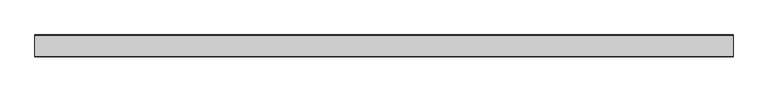
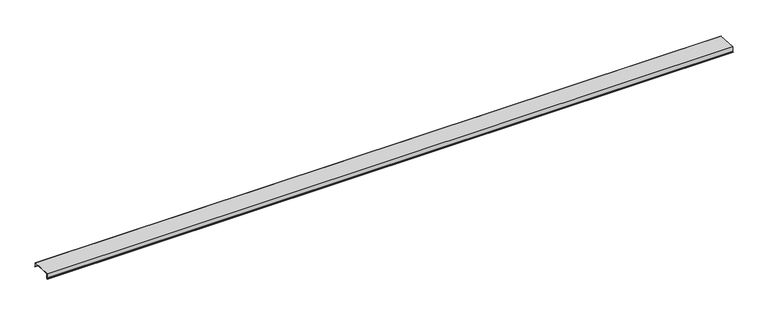
"""IFC4 building model written with IfcOpenShell, lengths in millimetres: proxy geometry, Generic Models 7:Generic Models 1:5:Generic Models 1:5 : Generic Models 7:Generic Models 1:337419:31 : Generic Models 7:Generic Models 1:5:Generic Models 1:5 : Generic Models 7:Generic Models 1:337419:311462."""

import ifcopenshell
import ifcopenshell.guid

model = None  # the IFC model being written
_history = None  # IfcOwnerHistory: only IFC2X3 demands one
_inside = {}  # id of a spatial element -> (the spatial element, [elements in it])
_under = {}  # id of a project, library or spatial element -> (it, [spatial elements below it])
_declared = {}  # id of a project -> (the project, [libraries it declares])
_typed = {}  # id of a type object -> (the type object, [elements of that type])
_made_of = {}  # id of a material, layer set ... -> (it, [elements and type objects made of it])


def new_model(schema):
    """Start an empty IFC model of exactly this schema.

    Asked for "IFC4X3", IfcOpenShell would pick the latest addendum, in which some entities
    have other attributes; the version numbers below select the first issue.
    IFC2X3 requires an IfcOwnerHistory on every rooted entity: one is made here for all.
    """
    global model, _history
    if schema == "IFC4X3":
        model = ifcopenshell.file(schema_version=(4, 3, 0, 0))
    else:
        model = ifcopenshell.file(schema=schema)
    _inside.clear()
    _under.clear()
    _declared.clear()
    _typed.clear()
    _made_of.clear()
    _history = None
    if model.schema == "IFC2X3":
        org = make("IfcOrganization", Name="unknown")
        user = make(
            "IfcPersonAndOrganization",
            ThePerson=make("IfcPerson", FamilyName="unknown"),
            TheOrganization=org,
        )
        app = make(
            "IfcApplication",
            ApplicationDeveloper=org,
            Version="unknown",
            ApplicationFullName="unknown",
            ApplicationIdentifier="unknown",
        )
        _history = make(
            "IfcOwnerHistory",
            OwningUser=user,
            OwningApplication=app,
            ChangeAction="ADDED",
            CreationDate=0,
        )
    return model


def make(cls, **values):
    """One entity of the class cls with the attributes given. An attribute that is None is left unset."""
    return model.create_entity(
        cls, **{name: value for name, value in values.items() if value is not None}
    )


def rooted(cls, **values):
    """An entity with a GlobalId (a new one), such as an element, a storey or a relation."""
    return make(cls, GlobalId=ifcopenshell.guid.new(), OwnerHistory=_history, **values)


def si_unit(unit_type, name, prefix=None):
    """IfcSIUnit, for example si_unit("LENGTHUNIT", "METRE", prefix="MILLI")."""
    return make("IfcSIUnit", UnitType=unit_type, Prefix=prefix, Name=name)


def assignment(units):
    """IfcUnitAssignment: the units of a project."""
    return None if units is None else make("IfcUnitAssignment", Units=units)


def point(xyz):
    """IfcCartesianPoint."""
    return None if xyz is None else make("IfcCartesianPoint", Coordinates=xyz)


def direction(xyz):
    """IfcDirection."""
    return None if xyz is None else make("IfcDirection", DirectionRatios=xyz)


def frame(location, z_axis=None, x_axis=None):
    """IfcAxis2Placement3D, a coordinate frame: its origin and axes. An axis left out is left unset."""
    return make(
        "IfcAxis2Placement3D",
        Location=point(location),
        Axis=direction(z_axis),
        RefDirection=direction(x_axis),
    )


def origin():
    """The frame at (0, 0, 0) with its axes left unset."""
    return frame((0.0, 0.0, 0.0))


def place(relative_to, where):
    """IfcLocalPlacement: puts the frame where relative to a parent placement (None: the world)."""
    return make(
        "IfcLocalPlacement", PlacementRelTo=relative_to, RelativePlacement=where
    )


def context(
    kind, dimensions, precision=None, world=None, true_north=None, identifier=None
):
    """IfcGeometricRepresentationContext, for example the 3D "Model" context."""
    return make(
        "IfcGeometricRepresentationContext",
        ContextIdentifier=identifier,
        ContextType=kind,
        CoordinateSpaceDimension=dimensions,
        Precision=precision,
        WorldCoordinateSystem=world,
        TrueNorth=true_north,
    )


def project(units=None, contexts=None):
    """IfcProject with its units and contexts."""
    return rooted(
        "IfcProject",
        Name="project",
        RepresentationContexts=contexts,
        UnitsInContext=assignment(units),
    )


def spatial(cls, under=None, at=None, **own):
    """A site, building, storey or space (cls), placed at a placement, below another one or the project."""
    s = rooted(cls, ObjectPlacement=at, **own)
    if under is not None:
        _under.setdefault(under.id(), (under, []))[1].append(s)
    return s


def polyline(points):
    """IfcPolyline through the points."""
    return make("IfcPolyline", Points=[point(p) for p in points])


def outline(outer, holes=None, kind="AREA"):
    """IfcArbitraryClosedProfileDef: a profile drawn as a closed curve; with holes, ...WithVoids."""
    if holes is None:
        return make("IfcArbitraryClosedProfileDef", ProfileType=kind, OuterCurve=outer)
    return make(
        "IfcArbitraryProfileDefWithVoids",
        ProfileType=kind,
        OuterCurve=outer,
        InnerCurves=holes,
    )


def extrude(swept, where, along, depth):
    """IfcExtrudedAreaSolid: the profile swept, set in the frame where, extruded along a direction by depth."""
    return make(
        "IfcExtrudedAreaSolid",
        SweptArea=swept,
        Position=where,
        ExtrudedDirection=direction(along),
        Depth=depth,
    )


def shape(context_of_items, identifier, shape_type, items):
    """IfcShapeRepresentation: the items that make up one representation, for example the "Body"."""
    return make(
        "IfcShapeRepresentation",
        ContextOfItems=context_of_items,
        RepresentationIdentifier=identifier,
        RepresentationType=shape_type,
        Items=items,
    )


def source(mapping_origin, context_of_items, identifier, shape_type, items):
    """IfcRepresentationMap: a shape defined once, which mapped items show again and again."""
    return make(
        "IfcRepresentationMap",
        MappingOrigin=mapping_origin,
        MappedRepresentation=shape(context_of_items, identifier, shape_type, items),
    )


def transform(
    local_origin,
    x_axis=None,
    y_axis=None,
    z_axis=None,
    scale=None,
    scale2=None,
    scale3=None,
    uniform=True,
):
    """IfcCartesianTransformationOperator3D, or its non-uniform kind. x_axis, y_axis, z_axis: its Axis1, 2, 3."""
    if uniform:
        return make(
            "IfcCartesianTransformationOperator3D",
            Axis1=direction(x_axis),
            Axis2=direction(y_axis),
            LocalOrigin=point(local_origin),
            Scale=scale,
            Axis3=direction(z_axis),
        )
    return make(
        "IfcCartesianTransformationOperator3DnonUniform",
        Axis1=direction(x_axis),
        Axis2=direction(y_axis),
        LocalOrigin=point(local_origin),
        Scale=scale,
        Axis3=direction(z_axis),
        Scale2=scale2,
        Scale3=scale3,
    )


def mapped(mapping_source, mapping_target):
    """IfcMappedItem: shows the shape of a source again, moved by a transform."""
    return make(
        "IfcMappedItem", MappingSource=mapping_source, MappingTarget=mapping_target
    )


def made_of(thing, what):
    """Note that an element or type object is made of a material, layer set ...; save() writes the relation."""
    if what is not None:
        _made_of.setdefault(what.id(), (what, []))[1].append(thing)
    return thing


def element(
    cls,
    number,
    at=None,
    inside=None,
    cuts=None,
    type_object=None,
    material=None,
    context=None,
    identifier="Body",
    shape_type=None,
    held_by="IfcProductDefinitionShape",
    body=None,
    shapes=None,
    **own,
):
    """One element of the class cls, such as IfcWall. Its Tag is "e" and its number.

    at: its placement. inside: the storey or other place that contains it. cuts: it is an
    opening in that element (IfcRelVoidsElement). A single representation is given by context,
    identifier, shape_type and body (its items); several are given by shapes. held_by: the class
    of the entity that holds the representations. save() writes the other relations.
    """
    e = rooted(cls, Tag="e%d" % number, ObjectPlacement=at, **own)
    if body is not None:
        shapes = [shape(context, identifier, shape_type, body)]
    if shapes is not None:
        e.Representation = make(held_by, Representations=shapes)
    if inside is not None:
        _inside.setdefault(inside.id(), (inside, []))[1].append(e)
    if cuts is not None:
        rooted(
            "IfcRelVoidsElement", RelatingBuildingElement=cuts, RelatedOpeningElement=e
        )
    if type_object is not None:
        _typed.setdefault(type_object.id(), (type_object, []))[1].append(e)
    return made_of(e, material)


def aggregate(whole, parts):
    """IfcRelAggregates: a whole, such as a stair, and the parts it consists of."""
    return rooted("IfcRelAggregates", RelatingObject=whole, RelatedObjects=parts)


def save(model, path):
    """Write the relations noted so far, then the file.

    IfcRelAggregates (storeys below a building ...), IfcRelContainedInSpatialStructure (elements
    in a storey), IfcRelDefinesByType, IfcRelAssociatesMaterial and IfcRelDeclares: one each for
    every whole, place, type object, material and project.
    """
    for whole, parts in _under.values():
        aggregate(whole, parts)
    for where, things in _inside.values():
        rooted(
            "IfcRelContainedInSpatialStructure",
            RelatedElements=things,
            RelatingStructure=where,
        )
    for kind, things in _typed.values():
        rooted("IfcRelDefinesByType", RelatedObjects=things, RelatingType=kind)
    for what, things in _made_of.values():
        rooted("IfcRelAssociatesMaterial", RelatedObjects=things, RelatingMaterial=what)
    for by, libraries in _declared.values():
        rooted("IfcRelDeclares", RelatingContext=by, RelatedDefinitions=libraries)
    model.write(path)


def generic_models_280975a4(model_context):
    return source(origin(), model_context, "Body", "SweptSolid", [
        extrude(outline(polyline([(-579111.8163841, 6099.8348677), (-579111.8163841, 6188.1524863), (-578729.2288841, 6168.101925), (-578729.2288841, 6099.8348677), (-578716.5288841, 6087.1348677), (-578717.6514161, 6086.0123357), (-578730.8163841, 6099.1773037), (-578730.8163841, 6166.5954438), (-579110.2288841, 6186.4796103), (-579110.2288841, 6099.1773037), (-579123.3938521, 6086.0123357), (-579124.5163841, 6087.1348677), (-579111.8163841, 6099.8348677)])), frame((790916.1132437, 0.0, 0.0), z_axis=(1.0, 0.0, 0.0), x_axis=(0.0, 1.0, 0.0)), (0.0, 0.0, 1.0), 12903.7635635),
    ])


if __name__ == "__main__":
    model = new_model("IFC4")
    model_context = context("Model", 3, world=origin())
    ifc_project = project(units=[si_unit("LENGTHUNIT", "METRE", prefix="MILLI")], contexts=[model_context])
    site = spatial("IfcSite", under=ifc_project)
    building = spatial("IfcBuilding", under=site)
    placement = place(None, origin())
    generic_models_shape = generic_models_280975a4(model_context)
    element("IfcBuildingElementProxy", 1, Name="Generic Models 7:Generic Models 1:5:Generic Models 1:5 : Generic Models 7:Generic Models 1:337419:31 : Generic Models 7:Generic Models 1:5:Generic Models 1:5 : Generic Models 7:Generic Models 1:337419:311462", ObjectType="Generic Models 7:Generic Models 1:5:Generic Models 1:5 : Generic Models 7:Generic Models 1:337419:31 : Generic Models 7:Generic Models 1:5:Generic Models 1:5 : Generic Models 7:Generic Models 1:337419:311462", at=placement, inside=building, context=model_context, shape_type="MappedRepresentation", body=[
        mapped(generic_models_shape, transform((0.0, 0.0, 0.0), x_axis=(1.0, 0.0, 0.0), y_axis=(0.0, 1.0, 0.0), z_axis=(0.0, 0.0, 1.0))),
    ])
    save(model, "model.ifc")

# Revit data of these elements
# Type "Generic Models 7:Generic Models 1:5:Generic Models 1:5 : Generic Models 7:Generic Models 1:337419:31 : Generic Models 7:Generic Models 1:5:Generic Models 1:5 : Generic Models 7:Generic Models 1:337419:311462"
#   NameOverride = "Generic Models 7:Generic Models 1:5:Generic Models 1:5 : Generic Models 7:Generic Models 1:337419:311462"
#   ObjectTypeOverride = "Generic Models 1:5 : Generic Models 7:Generic Models 1:337419"
#   Reference = "Generic Models 1"
#   Tag = "311462"
# Element 1 (IfcBuildingElementProxy, "Generic Models 7:Generic Models 1:5:Generic Models 1:5 : Generic Models 7:Generic Models 1:337419:31 : Generic Models 7:Generic Models 1:5:Generic Models 1:5 : Generic Models 7:Generic Models 1:337419:311462")
#   Materials on its faces: "SHEET METAL COPING (COLOR TO MATCH RESIN PANEL)"
# Materials
#   "SHEET METAL COPING (COLOR TO MATCH RESIN PANEL)": class "Generic", colour RGB 240 240 240, transparency 0, Keynote = "M07711300.01", Cost = 0
